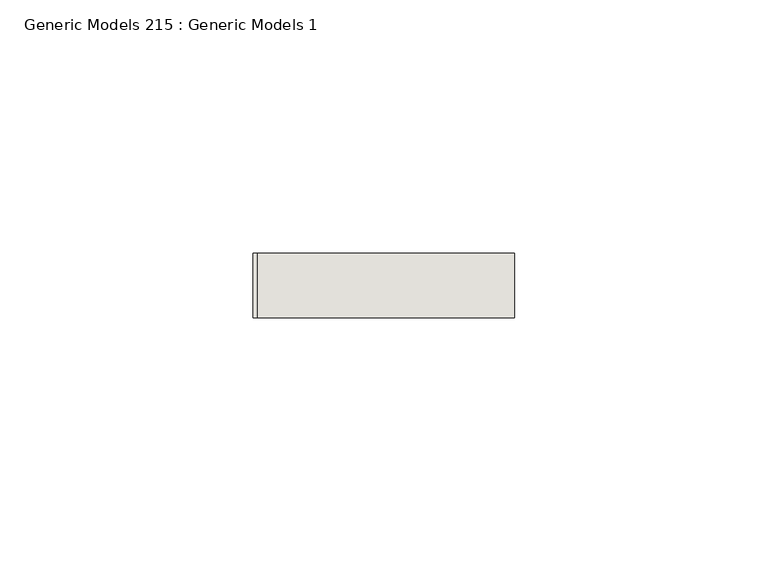
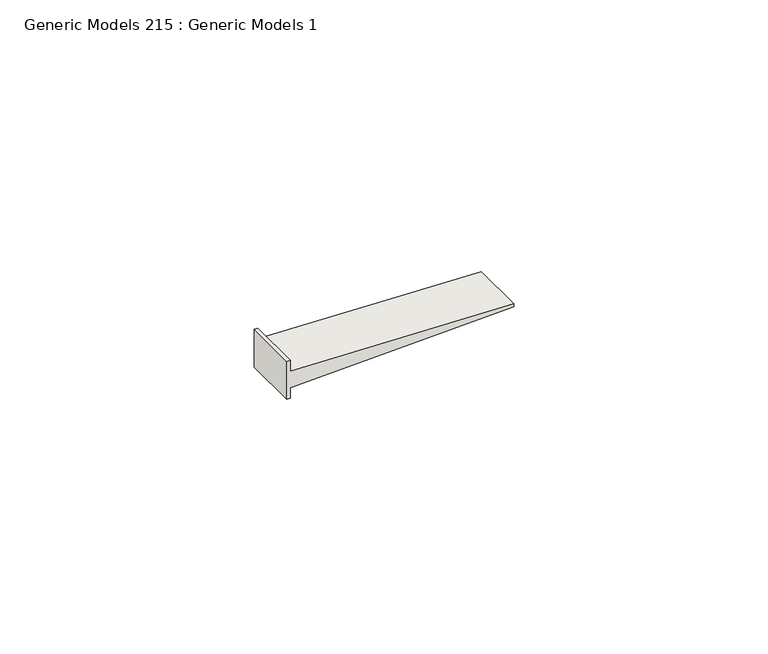
"""IFC4 building model written with IfcOpenShell, lengths in millimetres: wall geometry, Generic Models 215 : Generic Models 1."""

from ifc_helpers import new_model, si_unit, frame, origin, place, context, project, spatial, polyline, outline, extrude, source, transform, mapped, element, save


def generic_models_215_generic_models_1_2cccfb49(model_context):
    return source(origin(), model_context, "Body", "SweptSolid", [
        extrude(outline(polyline([(2409.6091, 780080.83125), (2400.5159, 780080.83125), (2400.5159, 780081.625), (2403.0657636, 780081.625), (2404.6631527, 780132.425), (2405.4618473, 780132.425), (2407.0592364, 780081.625), (2409.6091, 780081.625), (2409.6091, 780080.83125)])), frame((0.0, 565.15, 0.0), z_axis=(0.0, 1.0, 0.0), x_axis=(0.0, 0.0, 1.0)), (0.0, 0.0, 1.0), 12.7),
    ])


if __name__ == "__main__":
    model = new_model("IFC4")
    model_context = context("Model", 3, world=origin())
    ifc_project = project(units=[si_unit("LENGTHUNIT", "METRE", prefix="MILLI")], contexts=[model_context])
    site = spatial("IfcSite", under=ifc_project)
    building = spatial("IfcBuilding", under=site)
    placement = place(None, origin())
    generic_models_215_generic_models_1_shape = generic_models_215_generic_models_1_2cccfb49(model_context)
    element("IfcWall", 1, ObjectType="Generic Models 215 : Generic Models 1", at=placement, inside=building, context=model_context, shape_type="MappedRepresentation", body=[
        mapped(generic_models_215_generic_models_1_shape, transform((0.0, 0.0, 0.0), x_axis=(1.0, 0.0, 0.0), y_axis=(0.0, 1.0, 0.0), z_axis=(0.0, 0.0, 1.0))),
    ])
    save(model, "model.ifc")

# Revit data of these elements
# Element 1 (IfcWall, "Generic Models 215 : Generic Models 1")
#   Materials on its faces: "ATTACH GYPSUM BOARD TO STUDS AND NOT TO TOP TRACK"
# Materials
#   "ATTACH GYPSUM BOARD TO STUDS AND NOT TO TOP TRACK": class "Generic", colour RGB 48 48 48, transparency 0, Cost = 0
